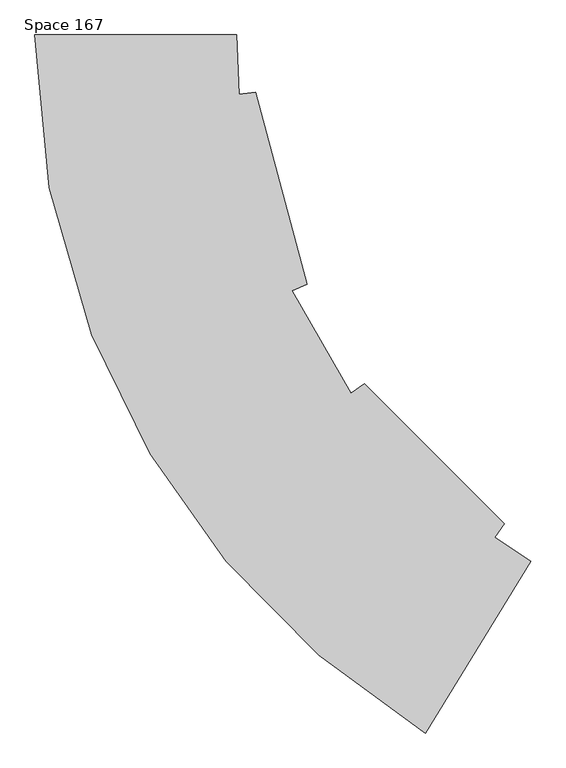
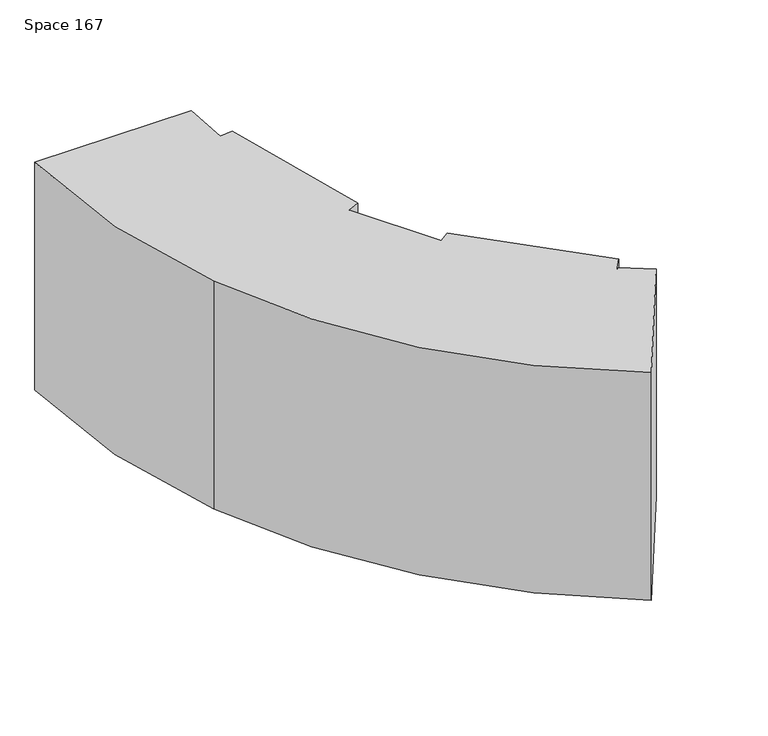
"""IFC4 building model written with IfcOpenShell, lengths in millimetres: proxy geometry, Space 167."""

from ifc_helpers import new_model, si_unit, point, frame_2d, origin, origin_with_axes, place, context, project, spatial, polyline, circle_curve, trimmed, segment, composite_curve, outline, extrude, source, transform, mapped, element, save


def space_167_e51e6080(model_context):
    return source(origin(), model_context, "Body", "SweptSolid", [
        extrude(outline(composite_curve([segment(trimmed(circle_curve(frame_2d((-24639.5440345, -26167.559635)), 8045.45), [point((-28843.280112, -33027.4334453))], [point((-32125.1720568, -29116.2269296))], False, "CARTESIAN"), True, "CONTINUOUS"), segment(trimmed(circle_curve(frame_2d((-24639.5440345, -26167.559635)), 8045.45), [point((-32125.1720568, -29116.2269296))], [point((-32684.9940345, -26167.559635))], False, "CARTESIAN"), True, "CONTINUOUS"), segment(polyline([(-32684.9940345, -26167.559635), (-30703.7940345, -26167.559635)]), True, "CONTINUOUS"), segment(trimmed(circle_curve(frame_2d((-24639.5440345, -26167.559635)), 6064.25), [point((-30703.7940345, -26167.559635))], [point((-30675.8754305, -26748.7922397))], True, "CARTESIAN"), True, "CONTINUOUS"), segment(polyline([(-30675.8754305, -26748.7922397), (-30515.399028, -26733.3401197), (-30011.0739702, -28615.5068591), (-30157.7766714, -28682.3631318)]), True, "CONTINUOUS"), segment(trimmed(circle_curve(frame_2d((-24639.5440345, -26167.559635)), 6064.25), [point((-30157.7766714, -28682.3631318))], [point((-29576.5440667, -29689.0875342))], True, "CARTESIAN"), True, "CONTINUOUS"), segment(polyline([(-29576.5440667, -29689.0875342), (-29445.2934855, -29595.4674045), (-28067.451804, -30973.309086), (-28161.0719337, -31104.5596672)]), True, "CONTINUOUS"), segment(trimmed(circle_curve(frame_2d((-24639.5440345, -26167.559635)), 6064.25), [point((-28161.0719337, -31104.5596672))], [point((-27808.1059556, -31338.1827517))], True, "CARTESIAN"), True, "CONTINUOUS"), segment(polyline([(-27808.1059556, -31338.1827517), (-28843.280112, -33027.4334453)]), True, "CONTINUOUS")], self_intersect=False)), origin_with_axes(), (0.0, 0.0, 1.0), 3048.0),
    ])


if __name__ == "__main__":
    model = new_model("IFC4")
    model_context = context("Model", 3, world=origin())
    ifc_project = project(units=[si_unit("LENGTHUNIT", "METRE", prefix="MILLI")], contexts=[model_context])
    site = spatial("IfcSite", under=ifc_project)
    building = spatial("IfcBuilding", under=site)
    placement = place(None, origin())
    space_167_shape = space_167_e51e6080(model_context)
    element("IfcBuildingElementProxy", 1, Name="Space 167", ObjectType="Space 167", at=placement, inside=building, context=model_context, shape_type="MappedRepresentation", body=[
        mapped(space_167_shape, transform((0.0, 0.0, 0.0), x_axis=(1.0, 0.0, 0.0), y_axis=(0.0, 1.0, 0.0), z_axis=(0.0, 0.0, 1.0))),
    ])
    save(model, "model.ifc")

# Revit data of these elements
# Element 1 (IfcBuildingElementProxy, "Space 167")
#   Materials on its faces: "Render Material 255-255-255"
# Materials
#   "Render Material 255-255-255": class "Unassigned", colour RGB 255 255 255, transparency 0
